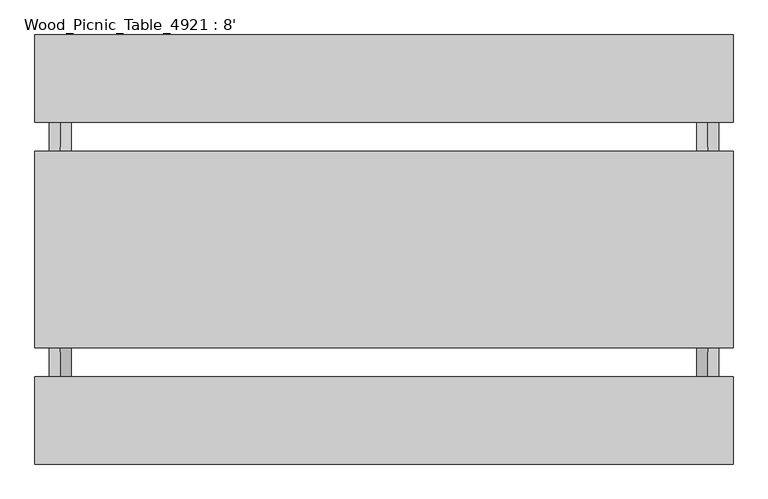
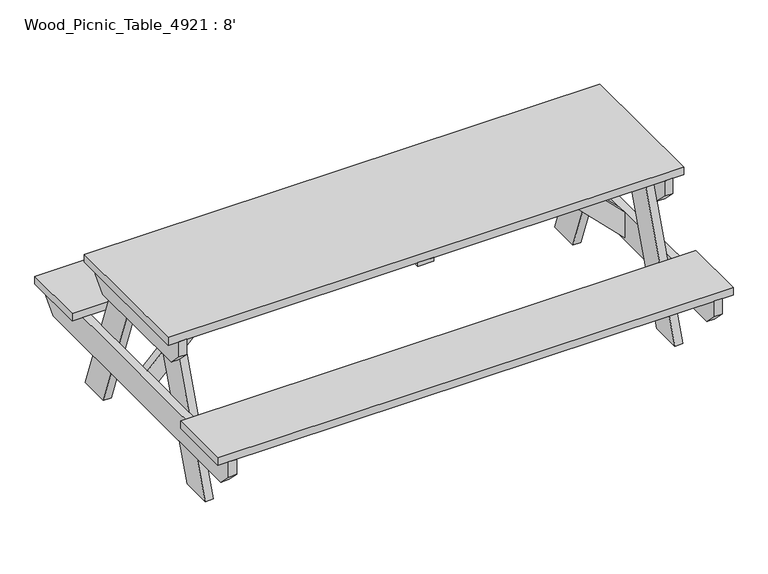
"""IFC4 building model written with IfcOpenShell, lengths in millimetres: furniture geometry, Wood_Picnic_Table_4921 : 8'."""

from ifc_helpers import new_model, si_unit, frame, origin, place, context, project, spatial, polyline, outline, extrude, source, transform, mapped, element, save


def wood_picnic_table_4921_8_f1337195(model_context):
    return source(origin(), model_context, "Body", "SweptSolid", [
        extrude(outline(polyline([(-79.8877235, 723.9), (-343.365776, 0.0), (-492.0314109, 0.0), (-228.5533583, 723.9), (-79.8877235, 723.9)])), frame((1092.2, 0.0, 0.0), z_axis=(1.0, 0.0, 0.0), x_axis=(0.0, 1.0, 0.0)), (0.0, 0.0, 1.0), 38.1),
        extrude(outline(polyline([(343.365776, 0.0), (79.8877235, 723.9), (228.5533583, 723.9), (492.0314109, 0.0), (343.365776, 0.0)])), frame((1092.2, 0.0, 0.0), z_axis=(1.0, 0.0, 0.0), x_axis=(0.0, 1.0, 0.0)), (0.0, 0.0, 1.0), 38.1),
        extrude(outline(polyline([(492.0314109, 0.0), (343.365776, 0.0), (79.8877235, 723.9), (228.5533583, 723.9), (492.0314109, 0.0)])), frame((-1130.3, 0.0, 0.0), z_axis=(1.0, 0.0, 0.0), x_axis=(0.0, 1.0, 0.0)), (0.0, 0.0, 1.0), 38.1),
        extrude(outline(polyline([(-492.0314109, 0.0), (-228.5533583, 723.9), (-79.8877235, 723.9), (-343.365776, 0.0), (-492.0314109, 0.0)])), frame((-1130.3, 0.0, 0.0), z_axis=(1.0, 0.0, 0.0), x_axis=(0.0, 1.0, 0.0)), (0.0, 0.0, 1.0), 38.1),
        extrude(outline(polyline([(723.9, 774.7), (723.9, 648.9764143), (242.5764143, 1130.3), (368.3, 1130.3), (723.9, 774.7)])), frame((0.0, -19.05, 0.0), z_axis=(0.0, 1.0, 0.0), x_axis=(0.0, 0.0, 1.0)), (0.0, 0.0, 1.0), 38.1),
        extrude(outline(polyline([(-749.3, 368.3), (749.3, 368.3), (749.3, 292.1), (685.8, 228.6), (-685.8, 228.6), (-749.3, 292.1), (-749.3, 368.3)])), frame((1130.3, 0.0, 0.0), z_axis=(1.0, 0.0, 0.0), x_axis=(0.0, 1.0, 0.0)), (0.0, 0.0, 1.0), 38.1),
        extrude(outline(polyline([(-342.9, 723.9), (342.9, 723.9), (342.9, 647.7), (279.4, 584.2), (-279.4, 584.2), (-342.9, 647.7), (-342.9, 723.9)])), frame((1130.3, 0.0, 0.0), z_axis=(1.0, 0.0, 0.0), x_axis=(0.0, 1.0, 0.0)), (0.0, 0.0, 1.0), 38.1),
        extrude(outline(polyline([(38.1, -342.9), (-38.1, -342.9), (-38.1, 342.9), (38.1, 342.9), (38.1, -342.9)])), frame((0.0, 0.0, 704.85), z_axis=(0.0, 0.0, 1.0), x_axis=(1.0, 0.0, 0.0)), (0.0, 0.0, 1.0), 19.05),
        extrude(outline(polyline([(723.9, -774.7), (368.3, -1130.3), (242.5764143, -1130.3), (723.9, -648.9764143), (723.9, -774.7)])), frame((0.0, -19.05, 0.0), z_axis=(0.0, 1.0, 0.0), x_axis=(0.0, 0.0, 1.0)), (0.0, 0.0, 1.0), 38.1),
        extrude(outline(polyline([(749.3, 292.1), (685.8, 228.6), (-685.8, 228.6), (-749.3, 292.1), (-749.3, 368.3), (749.3, 368.3), (749.3, 292.1)])), frame((-1168.4, 0.0, 0.0), z_axis=(1.0, 0.0, 0.0), x_axis=(0.0, 1.0, 0.0)), (0.0, 0.0, 1.0), 38.1),
        extrude(outline(polyline([(342.9, 647.7), (279.4, 584.2), (-279.4, 584.2), (-342.9, 647.7), (-342.9, 723.9), (342.9, 723.9), (342.9, 647.7)])), frame((-1168.4, 0.0, 0.0), z_axis=(1.0, 0.0, 0.0), x_axis=(0.0, 1.0, 0.0)), (0.0, 0.0, 1.0), 38.1),
        extrude(outline(polyline([(1219.2, 749.3), (1219.2, 444.5), (-1219.2, 444.5), (-1219.2, 749.3), (1219.2, 749.3)])), frame((0.0, 0.0, 368.3), z_axis=(0.0, 0.0, 1.0), x_axis=(1.0, 0.0, 0.0)), (0.0, 0.0, 1.0), 38.1),
        extrude(outline(polyline([(1219.2, -444.5), (1219.2, -749.3), (-1219.2, -749.3), (-1219.2, -444.5), (1219.2, -444.5)])), frame((0.0, 0.0, 368.3), z_axis=(0.0, 0.0, 1.0), x_axis=(1.0, 0.0, 0.0)), (0.0, 0.0, 1.0), 38.1),
        extrude(outline(polyline([(1219.2, 342.9), (1219.2, -342.9), (-1219.2, -342.9), (-1219.2, 342.9), (1219.2, 342.9)])), frame((0.0, 0.0, 723.9), z_axis=(0.0, 0.0, 1.0), x_axis=(1.0, 0.0, 0.0)), (0.0, 0.0, 1.0), 38.1),
    ])


if __name__ == "__main__":
    model = new_model("IFC4")
    model_context = context("Model", 3, world=origin())
    ifc_project = project(units=[si_unit("LENGTHUNIT", "METRE", prefix="MILLI")], contexts=[model_context])
    site = spatial("IfcSite", under=ifc_project)
    building = spatial("IfcBuilding", under=site)
    placement = place(None, origin())
    wood_picnic_table_4921_8_shape = wood_picnic_table_4921_8_f1337195(model_context)
    element("IfcFurniture", 1, ObjectType="Wood_Picnic_Table_4921 : 8'", at=placement, inside=building, context=model_context, shape_type="MappedRepresentation", body=[
        mapped(wood_picnic_table_4921_8_shape, transform((0.0, 0.0, 0.0), x_axis=(1.0, 0.0, 0.0), y_axis=(0.0, 1.0, 0.0), z_axis=(0.0, 0.0, 1.0))),
    ])
    save(model, "model.ifc")

# Revit data of these elements
# Type "Wood_Picnic_Table_4921 : 8'"
#   Length = 2.4384 m
#   Seating = 8
#   Render Material = Wood - Yellow Pine
#   Default Elevation = 0
# Element 1 (IfcFurniture, "Wood_Picnic_Table_4921 : 8'")
#   Materials on its faces: "Wood - Yellow Pine"
# Materials
#   "Wood - Yellow Pine": class "Wood", colour RGB 173 129 56, transparency 0, Description = "Cherry"
